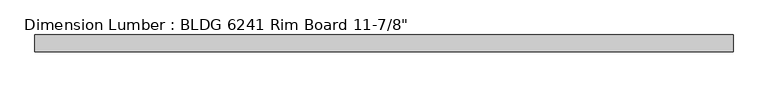
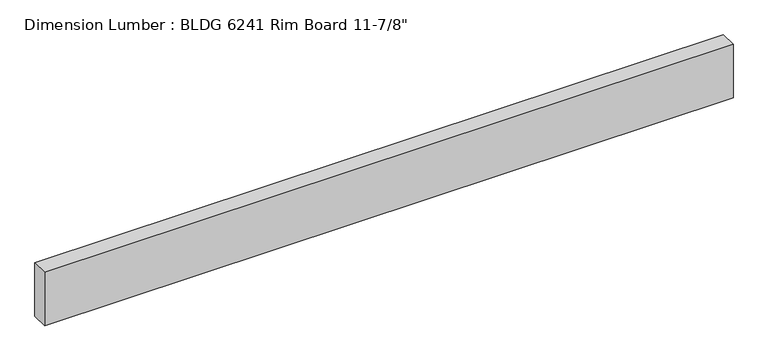
"""IFC4 building model written with IfcOpenShell, lengths in millimetres: beam geometry."""

from ifc_helpers import new_model, si_unit, frame, origin, place, context, project, spatial, polyline, outline, extrude, source, transform, mapped, element, save


def beam_9835caef(model_context):
    return source(origin(), model_context, "Body", "SweptSolid", [
        extrude(outline(polyline([(1815.7808964, 44.45), (1815.7808964, -44.45), (-1860.2308964, -44.45), (-1860.2308964, 44.45), (1815.7808964, 44.45)])), frame((0.0, 0.0, -150.8125), z_axis=(0.0, 0.0, 1.0), x_axis=(1.0, 0.0, 0.0)), (0.0, 0.0, 1.0), 301.625),
    ])


if __name__ == "__main__":
    model = new_model("IFC4")
    model_context = context("Model", 3, world=origin())
    ifc_project = project(units=[si_unit("LENGTHUNIT", "METRE", prefix="MILLI")], contexts=[model_context])
    site = spatial("IfcSite", under=ifc_project)
    building = spatial("IfcBuilding", under=site)
    placement = place(None, origin())
    beam_shape = beam_9835caef(model_context)
    element("IfcBeam", 1, ObjectType="Dimension Lumber : BLDG 6241 Rim Board 11-7/8\"", at=placement, inside=building, context=model_context, shape_type="MappedRepresentation", body=[
        mapped(beam_shape, transform((0.0, 0.0, 0.0), x_axis=(1.0, 0.0, 0.0), y_axis=(0.0, 1.0, 0.0), z_axis=(0.0, 0.0, 1.0))),
    ])
    save(model, "model.ifc")

# Revit data of these elements
# Type "Dimension Lumber : BLDG 6241 Rim Board 11-7/8\""
#   Assembly Code = "B10"
#   A = 0.273472 SF
#   Length [instance default] = 5' - 0"
#   b = 0' - 3 1/2"
#   d = 0' - 11 7/8"
#   Structural Material [instance default] = Softwood, Lumber
# Element 1 (IfcBeam, "Dimension Lumber : BLDG 6241 Rim Board 11-7/8\"")
#   Materials on its faces: "Softwood, Lumber"
# Materials
#   "Softwood, Lumber": class "Wood", colour RGB 223 192 134, transparency 0, Description = "Pinus Echinata", Cost = 0
